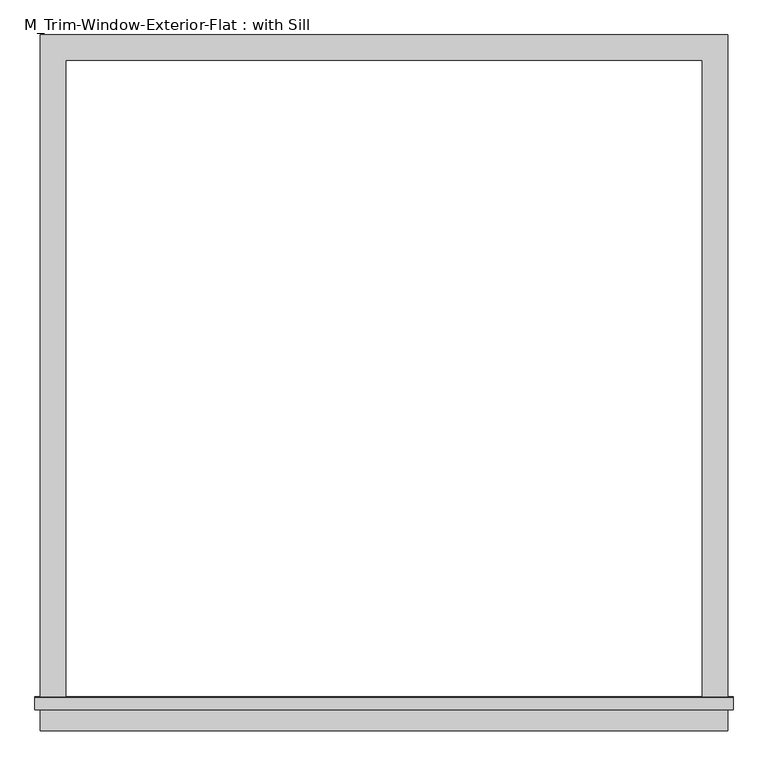
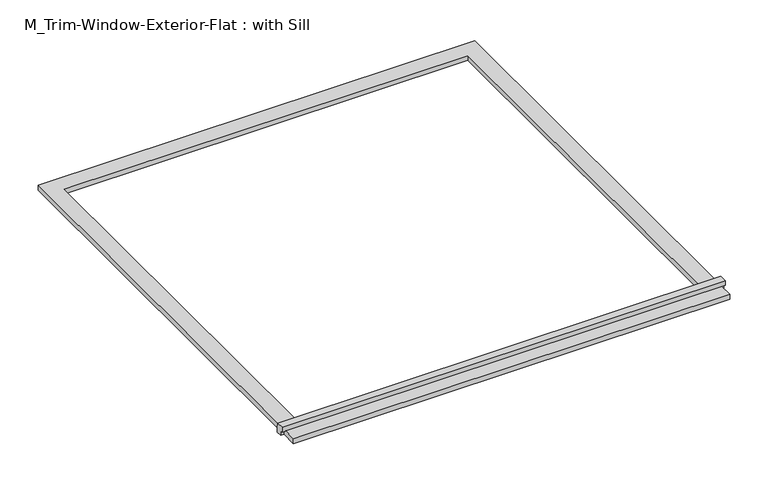
"""IFC4 building model written with IfcOpenShell, lengths in millimetres: proxy geometry, M_Trim-Window-Exterior-Flat : with Sill."""

from ifc_helpers import new_model, si_unit, frame, origin, origin_with_axes, place, context, project, spatial, polyline, outline, extrude, source, transform, mapped, element, save


def m_trim_window_exterior_flat_with_sill_22923e22(model_context):
    return source(origin(), model_context, "Body", "SweptSolid", [
        extrude(outline(polyline([(810.0, -1520.4323709), (810.0, -1580.4323709), (-810.0, -1580.4323709), (-810.0, -1520.4323709), (810.0, -1520.4323709)])), origin_with_axes(), (0.0, 0.0, 1.0), 19.05),
        extrude(outline(polyline([(-1530.0, 38.1), (-1502.4580645, 38.1), (-1500.0, 19.05), (-1500.0, 0.0), (-1520.4323709, 0.0), (-1520.4323709, 19.05), (-1530.0, 19.05), (-1530.0, 38.1)])), frame((-822.7, 0.0, 0.0), z_axis=(1.0, 0.0, 0.0), x_axis=(0.0, 1.0, 0.0)), (0.0, 0.0, 1.0), 1645.4),
        extrude(outline(polyline([(-810.0, 60.0), (810.0, 60.0), (810.0, -1500.0), (750.0, -1500.0), (750.0, 0.0), (-750.0, 0.0), (-750.0, -1500.0), (-810.0, -1500.0), (-810.0, 60.0)])), origin_with_axes(), (0.0, 0.0, 1.0), 19.05),
    ])


if __name__ == "__main__":
    model = new_model("IFC4")
    model_context = context("Model", 3, world=origin())
    ifc_project = project(units=[si_unit("LENGTHUNIT", "METRE", prefix="MILLI")], contexts=[model_context])
    site = spatial("IfcSite", under=ifc_project)
    building = spatial("IfcBuilding", under=site)
    placement = place(None, origin())
    m_trim_window_exterior_flat_with_sill_shape = m_trim_window_exterior_flat_with_sill_22923e22(model_context)
    element("IfcBuildingElementProxy", 1, Name="M_Trim-Window-Exterior-Flat : with Sill", ObjectType="M_Trim-Window-Exterior-Flat : with Sill", at=placement, inside=building, context=model_context, shape_type="MappedRepresentation", body=[
        mapped(m_trim_window_exterior_flat_with_sill_shape, transform((0.0, 0.0, 0.0), x_axis=(1.0, 0.0, 0.0), y_axis=(0.0, 1.0, 0.0), z_axis=(0.0, 0.0, 1.0))),
    ])
    save(model, "model.ifc")

# Revit data of these elements
# Type "M_Trim-Window-Exterior-Flat : with Sill"
#   Trim Width = 0.06 m
#   Trim Thickness_Picture Frame = 0.03 m
#   Trim Thickness_with Sill = 0.01905 m
#   Sill Thickness = 0.03 m
#   Opening Width [instance default] = 0.6 m
#   Opening Height [instance default] = 0.9 m
#   Default Elevation = 1.2 m
#   Sill = yes
#   Picture Frame = no
#   Trim Material [instance default] = none
# Element 1 (IfcBuildingElementProxy, "M_Trim-Window-Exterior-Flat : with Sill")
#   Opening Width = 1.5 m
#   Opening Height = 1.5 m
#   Trim Material = Clad - White
#   Materials on its faces: "Clad - White"
# Materials
#   "Clad - White": class "Wood", colour RGB 242 242 238, transparency 0, Cost = 0
